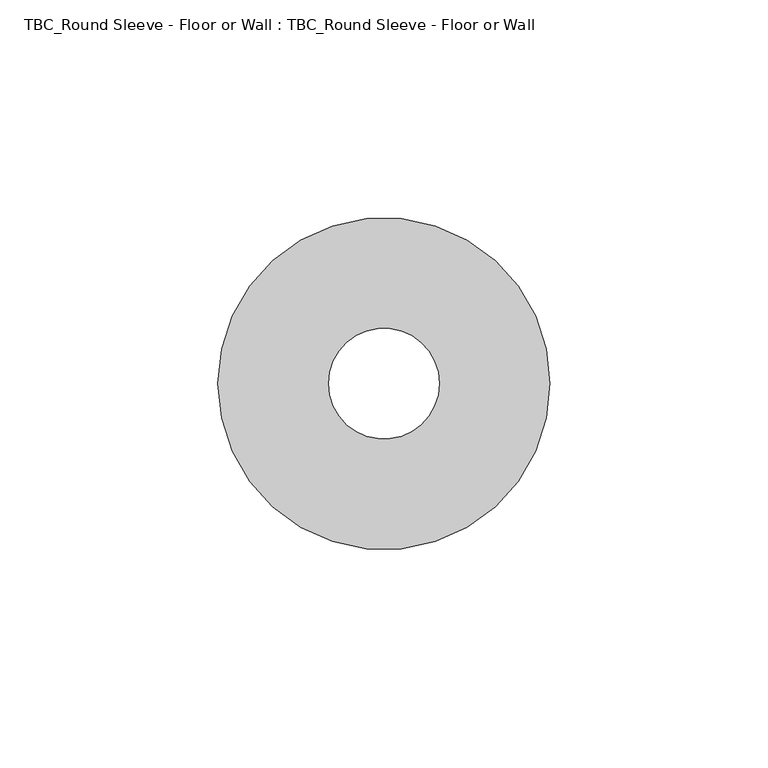
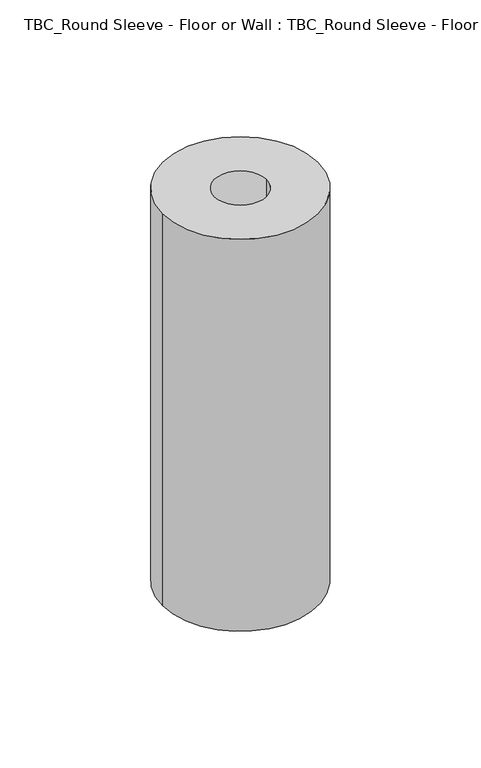
"""IFC4 building model written with IfcOpenShell, lengths in millimetres: proxy geometry, TBC_Round Sleeve - Floor or Wall : TBC_Round Sleeve - Floor or Wall."""

from ifc_helpers import new_model, si_unit, point, frame, origin, origin_2d, place, context, project, spatial, circle_curve, trimmed, segment, composite_curve, outline, extrude, source, transform, mapped, element, save


def tbc_round_sleeve_floor_or_wall_tbc_round_sleeve_floor_or_90b5a73a(model_context):
    return source(origin(), model_context, "Body", "SweptSolid", [
        extrude(outline(composite_curve([segment(trimmed(circle_curve(origin_2d(), 38.1), [point((-38.1, 0.0))], [point((38.1, 0.0))], False, "CARTESIAN"), True, "CONTINUOUS"), segment(trimmed(circle_curve(origin_2d(), 38.1), [point((38.1, 0.0))], [point((-38.1, 0.0))], False, "CARTESIAN"), True, "CONTINUOUS")], self_intersect=False), holes=[composite_curve([segment(trimmed(circle_curve(origin_2d(), 12.7), [point((-12.7, 0.0))], [point((12.7, 0.0))], True, "CARTESIAN"), True, "CONTINUOUS"), segment(trimmed(circle_curve(origin_2d(), 12.7), [point((12.7, 0.0))], [point((-12.7, 0.0))], True, "CARTESIAN"), True, "CONTINUOUS")], self_intersect=False)]), frame((0.0, 0.0, -203.2), z_axis=(0.0, 0.0, 1.0), x_axis=(1.0, 0.0, 0.0)), (0.0, 0.0, 1.0), 203.2),
    ])


if __name__ == "__main__":
    model = new_model("IFC4")
    model_context = context("Model", 3, world=origin())
    ifc_project = project(units=[si_unit("LENGTHUNIT", "METRE", prefix="MILLI")], contexts=[model_context])
    site = spatial("IfcSite", under=ifc_project)
    building = spatial("IfcBuilding", under=site)
    placement = place(None, origin())
    tbc_round_sleeve_floor_or_wall_tbc_round_sleeve_floor_or_shape = tbc_round_sleeve_floor_or_wall_tbc_round_sleeve_floor_or_90b5a73a(model_context)
    element("IfcBuildingElementProxy", 1, Name="TBC_Round Sleeve - Floor or Wall : TBC_Round Sleeve - Floor or Wall", ObjectType="TBC_Round Sleeve - Floor or Wall : TBC_Round Sleeve - Floor or Wall", at=placement, inside=building, context=model_context, shape_type="MappedRepresentation", body=[
        mapped(tbc_round_sleeve_floor_or_wall_tbc_round_sleeve_floor_or_shape, transform((0.0, 0.0, 0.0), x_axis=(1.0, 0.0, 0.0), y_axis=(0.0, 1.0, 0.0), z_axis=(0.0, 0.0, 1.0))),
    ])
    save(model, "model.ifc")

# Revit data of these elements
# Type "TBC_Round Sleeve - Floor or Wall : TBC_Round Sleeve - Floor or Wall"
#   Tag Dimension [instance default] = ""
#   MEP Type [instance default] = ""
#   MEP Element [instance default] = ""
#   MEP Category [instance default] = ""
#   Host Element Type [instance default] = ""
#   Host Element Id [instance default] = ""
#   Host Element Category [instance default] = ""
#   Control Line Y [instance default] = ""
#   Control Line X [instance default] = ""
#   Sleeve Radius [instance default] = 1' - 0"
#   Sleeve Edge [instance default] = 1' - 2"
#   Sleeve Depth [instance default] = 3' - 0"
#   Distance Y [instance default] = 0' - 0"
#   Distance X [instance default] = 0' - 0"
#   Default Elevation = 0
# Element 1 (IfcBuildingElementProxy, "TBC_Round Sleeve - Floor or Wall : TBC_Round Sleeve - Floor or Wall")
#   Tag Dimension = "3\""
#   MEP Type = "Mechanical-COND"
#   MEP Element = "898696"
#   MEP Category = "Pipe"
#   Host Element Type = "8\" Plank"
#   Host Element Id = "529506"
#   Host Element Category = "Floors"
#   Sleeve Radius = 0' - 1"
#   Sleeve Edge = 0' - 3"
#   Sleeve Depth = 0' - 8"
